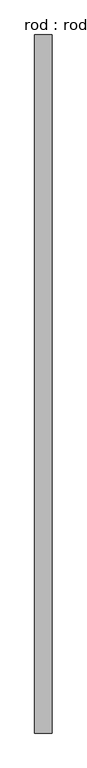
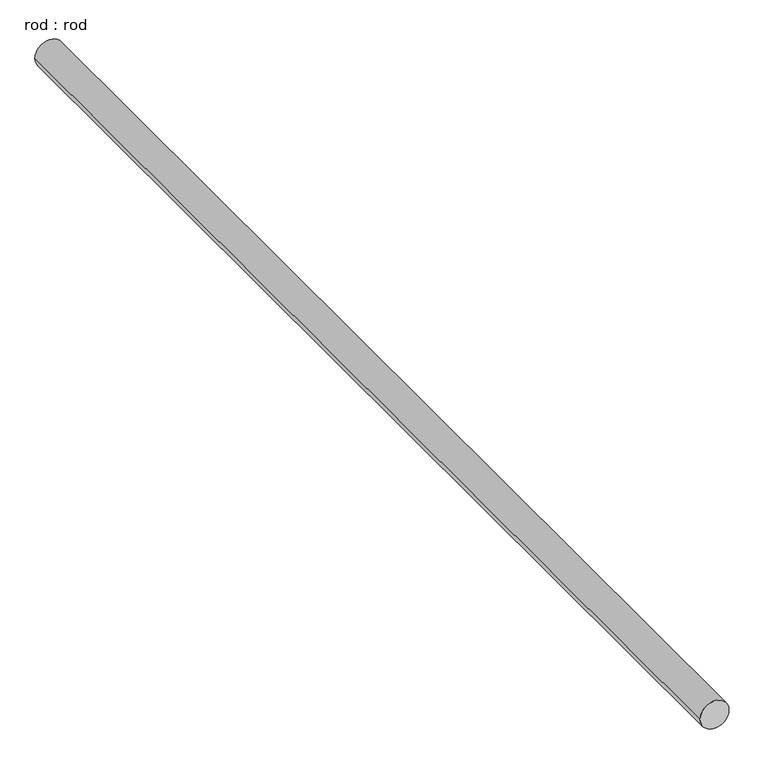
"""IFC4 building model written with IfcOpenShell, lengths in millimetres: proxy geometry, rod : rod."""

from ifc_helpers import new_model, si_unit, point, frame, frame_2d, origin, place, context, project, spatial, circle_curve, trimmed, segment, composite_curve, outline, extrude, source, transform, mapped, element, save


def rod_rod_87fd5f93(model_context):
    return source(origin(), model_context, "Body", "SweptSolid", [
        extrude(outline(composite_curve([segment(trimmed(circle_curve(frame_2d((0.0108462, 0.0)), 200.0), [point((0.0108462, 200.0))], [point((0.0108462, -200.0))], False, "CARTESIAN"), True, "CONTINUOUS"), segment(trimmed(circle_curve(frame_2d((0.0108462, 0.0)), 200.0), [point((0.0108462, -200.0))], [point((0.0108462, 200.0))], False, "CARTESIAN"), True, "CONTINUOUS")], self_intersect=False)), frame((0.0, -3862.6285275, 0.0), z_axis=(0.0, 1.0, 0.0), x_axis=(0.0, 0.0, 1.0)), (0.0, 0.0, 1.0), 15910.7142857),
    ])


if __name__ == "__main__":
    model = new_model("IFC4")
    model_context = context("Model", 3, world=origin())
    ifc_project = project(units=[si_unit("LENGTHUNIT", "METRE", prefix="MILLI")], contexts=[model_context])
    site = spatial("IfcSite", under=ifc_project)
    building = spatial("IfcBuilding", under=site)
    placement = place(None, origin())
    rod_rod_shape = rod_rod_87fd5f93(model_context)
    element("IfcBuildingElementProxy", 1, Name="rod : rod", ObjectType="rod : rod", at=placement, inside=building, context=model_context, shape_type="MappedRepresentation", body=[
        mapped(rod_rod_shape, transform((0.0, 0.0, 0.0), x_axis=(1.0, 0.0, 0.0), y_axis=(0.0, 1.0, 0.0), z_axis=(0.0, 0.0, 1.0))),
    ])
    save(model, "model.ifc")

# Revit data of these elements
# Type "rod : rod"
#   Default Elevation = 0
